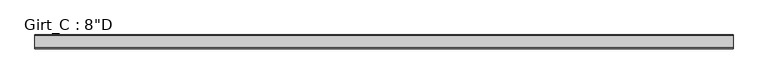
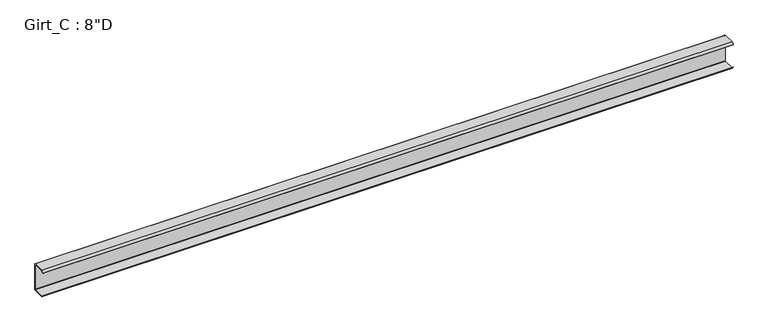
"""IFC4 building model written with IfcOpenShell, lengths in millimetres: beam geometry."""

import ifcopenshell
import ifcopenshell.guid

model = None  # the IFC model being written
_history = None  # IfcOwnerHistory: only IFC2X3 demands one
_inside = {}  # id of a spatial element -> (the spatial element, [elements in it])
_under = {}  # id of a project, library or spatial element -> (it, [spatial elements below it])
_declared = {}  # id of a project -> (the project, [libraries it declares])
_typed = {}  # id of a type object -> (the type object, [elements of that type])
_made_of = {}  # id of a material, layer set ... -> (it, [elements and type objects made of it])


def new_model(schema):
    """Start an empty IFC model of exactly this schema.

    Asked for "IFC4X3", IfcOpenShell would pick the latest addendum, in which some entities
    have other attributes; the version numbers below select the first issue.
    IFC2X3 requires an IfcOwnerHistory on every rooted entity: one is made here for all.
    """
    global model, _history
    if schema == "IFC4X3":
        model = ifcopenshell.file(schema_version=(4, 3, 0, 0))
    else:
        model = ifcopenshell.file(schema=schema)
    _inside.clear()
    _under.clear()
    _declared.clear()
    _typed.clear()
    _made_of.clear()
    _history = None
    if model.schema == "IFC2X3":
        org = make("IfcOrganization", Name="unknown")
        user = make(
            "IfcPersonAndOrganization",
            ThePerson=make("IfcPerson", FamilyName="unknown"),
            TheOrganization=org,
        )
        app = make(
            "IfcApplication",
            ApplicationDeveloper=org,
            Version="unknown",
            ApplicationFullName="unknown",
            ApplicationIdentifier="unknown",
        )
        _history = make(
            "IfcOwnerHistory",
            OwningUser=user,
            OwningApplication=app,
            ChangeAction="ADDED",
            CreationDate=0,
        )
    return model


def make(cls, **values):
    """One entity of the class cls with the attributes given. An attribute that is None is left unset."""
    return model.create_entity(
        cls, **{name: value for name, value in values.items() if value is not None}
    )


def rooted(cls, **values):
    """An entity with a GlobalId (a new one), such as an element, a storey or a relation."""
    return make(cls, GlobalId=ifcopenshell.guid.new(), OwnerHistory=_history, **values)


def si_unit(unit_type, name, prefix=None):
    """IfcSIUnit, for example si_unit("LENGTHUNIT", "METRE", prefix="MILLI")."""
    return make("IfcSIUnit", UnitType=unit_type, Prefix=prefix, Name=name)


def assignment(units):
    """IfcUnitAssignment: the units of a project."""
    return None if units is None else make("IfcUnitAssignment", Units=units)


def point(xyz):
    """IfcCartesianPoint."""
    return None if xyz is None else make("IfcCartesianPoint", Coordinates=xyz)


def direction(xyz):
    """IfcDirection."""
    return None if xyz is None else make("IfcDirection", DirectionRatios=xyz)


def frame(location, z_axis=None, x_axis=None):
    """IfcAxis2Placement3D, a coordinate frame: its origin and axes. An axis left out is left unset."""
    return make(
        "IfcAxis2Placement3D",
        Location=point(location),
        Axis=direction(z_axis),
        RefDirection=direction(x_axis),
    )


def frame_2d(location, x_axis=None):
    """IfcAxis2Placement2D, a coordinate frame in the plane: its origin and x axis."""
    return make(
        "IfcAxis2Placement2D", Location=point(location), RefDirection=direction(x_axis)
    )


def origin():
    """The frame at (0, 0, 0) with its axes left unset."""
    return frame((0.0, 0.0, 0.0))


def place(relative_to, where):
    """IfcLocalPlacement: puts the frame where relative to a parent placement (None: the world)."""
    return make(
        "IfcLocalPlacement", PlacementRelTo=relative_to, RelativePlacement=where
    )


def context(
    kind, dimensions, precision=None, world=None, true_north=None, identifier=None
):
    """IfcGeometricRepresentationContext, for example the 3D "Model" context."""
    return make(
        "IfcGeometricRepresentationContext",
        ContextIdentifier=identifier,
        ContextType=kind,
        CoordinateSpaceDimension=dimensions,
        Precision=precision,
        WorldCoordinateSystem=world,
        TrueNorth=true_north,
    )


def project(units=None, contexts=None):
    """IfcProject with its units and contexts."""
    return rooted(
        "IfcProject",
        Name="project",
        RepresentationContexts=contexts,
        UnitsInContext=assignment(units),
    )


def spatial(cls, under=None, at=None, **own):
    """A site, building, storey or space (cls), placed at a placement, below another one or the project."""
    s = rooted(cls, ObjectPlacement=at, **own)
    if under is not None:
        _under.setdefault(under.id(), (under, []))[1].append(s)
    return s


def polyline(points):
    """IfcPolyline through the points."""
    return make("IfcPolyline", Points=[point(p) for p in points])


def circle_curve(where, radius):
    """IfcCircle in the frame where."""
    return make("IfcCircle", Position=where, Radius=radius)


def trimmed(basis, trim1, trim2, sense, master):
    """IfcTrimmedCurve: the piece of a basis curve between two trims."""
    return make(
        "IfcTrimmedCurve",
        BasisCurve=basis,
        Trim1=trim1,
        Trim2=trim2,
        SenseAgreement=sense,
        MasterRepresentation=master,
    )


def segment(curve, same_sense, transition):
    """IfcCompositeCurveSegment."""
    return make(
        "IfcCompositeCurveSegment",
        Transition=transition,
        SameSense=same_sense,
        ParentCurve=curve,
    )


def composite_curve(segments, self_intersect=None):
    """IfcCompositeCurve: segments joined end to end."""
    return make("IfcCompositeCurve", Segments=segments, SelfIntersect=self_intersect)


def outline(outer, holes=None, kind="AREA"):
    """IfcArbitraryClosedProfileDef: a profile drawn as a closed curve; with holes, ...WithVoids."""
    if holes is None:
        return make("IfcArbitraryClosedProfileDef", ProfileType=kind, OuterCurve=outer)
    return make(
        "IfcArbitraryProfileDefWithVoids",
        ProfileType=kind,
        OuterCurve=outer,
        InnerCurves=holes,
    )


def extrude(swept, where, along, depth):
    """IfcExtrudedAreaSolid: the profile swept, set in the frame where, extruded along a direction by depth."""
    return make(
        "IfcExtrudedAreaSolid",
        SweptArea=swept,
        Position=where,
        ExtrudedDirection=direction(along),
        Depth=depth,
    )


def shape(context_of_items, identifier, shape_type, items):
    """IfcShapeRepresentation: the items that make up one representation, for example the "Body"."""
    return make(
        "IfcShapeRepresentation",
        ContextOfItems=context_of_items,
        RepresentationIdentifier=identifier,
        RepresentationType=shape_type,
        Items=items,
    )


def source(mapping_origin, context_of_items, identifier, shape_type, items):
    """IfcRepresentationMap: a shape defined once, which mapped items show again and again."""
    return make(
        "IfcRepresentationMap",
        MappingOrigin=mapping_origin,
        MappedRepresentation=shape(context_of_items, identifier, shape_type, items),
    )


def transform(
    local_origin,
    x_axis=None,
    y_axis=None,
    z_axis=None,
    scale=None,
    scale2=None,
    scale3=None,
    uniform=True,
):
    """IfcCartesianTransformationOperator3D, or its non-uniform kind. x_axis, y_axis, z_axis: its Axis1, 2, 3."""
    if uniform:
        return make(
            "IfcCartesianTransformationOperator3D",
            Axis1=direction(x_axis),
            Axis2=direction(y_axis),
            LocalOrigin=point(local_origin),
            Scale=scale,
            Axis3=direction(z_axis),
        )
    return make(
        "IfcCartesianTransformationOperator3DnonUniform",
        Axis1=direction(x_axis),
        Axis2=direction(y_axis),
        LocalOrigin=point(local_origin),
        Scale=scale,
        Axis3=direction(z_axis),
        Scale2=scale2,
        Scale3=scale3,
    )


def mapped(mapping_source, mapping_target):
    """IfcMappedItem: shows the shape of a source again, moved by a transform."""
    return make(
        "IfcMappedItem", MappingSource=mapping_source, MappingTarget=mapping_target
    )


def made_of(thing, what):
    """Note that an element or type object is made of a material, layer set ...; save() writes the relation."""
    if what is not None:
        _made_of.setdefault(what.id(), (what, []))[1].append(thing)
    return thing


def element(
    cls,
    number,
    at=None,
    inside=None,
    cuts=None,
    type_object=None,
    material=None,
    context=None,
    identifier="Body",
    shape_type=None,
    held_by="IfcProductDefinitionShape",
    body=None,
    shapes=None,
    **own,
):
    """One element of the class cls, such as IfcWall. Its Tag is "e" and its number.

    at: its placement. inside: the storey or other place that contains it. cuts: it is an
    opening in that element (IfcRelVoidsElement). A single representation is given by context,
    identifier, shape_type and body (its items); several are given by shapes. held_by: the class
    of the entity that holds the representations. save() writes the other relations.
    """
    e = rooted(cls, Tag="e%d" % number, ObjectPlacement=at, **own)
    if body is not None:
        shapes = [shape(context, identifier, shape_type, body)]
    if shapes is not None:
        e.Representation = make(held_by, Representations=shapes)
    if inside is not None:
        _inside.setdefault(inside.id(), (inside, []))[1].append(e)
    if cuts is not None:
        rooted(
            "IfcRelVoidsElement", RelatingBuildingElement=cuts, RelatedOpeningElement=e
        )
    if type_object is not None:
        _typed.setdefault(type_object.id(), (type_object, []))[1].append(e)
    return made_of(e, material)


def aggregate(whole, parts):
    """IfcRelAggregates: a whole, such as a stair, and the parts it consists of."""
    return rooted("IfcRelAggregates", RelatingObject=whole, RelatedObjects=parts)


def save(model, path):
    """Write the relations noted so far, then the file.

    IfcRelAggregates (storeys below a building ...), IfcRelContainedInSpatialStructure (elements
    in a storey), IfcRelDefinesByType, IfcRelAssociatesMaterial and IfcRelDeclares: one each for
    every whole, place, type object, material and project.
    """
    for whole, parts in _under.values():
        aggregate(whole, parts)
    for where, things in _inside.values():
        rooted(
            "IfcRelContainedInSpatialStructure",
            RelatedElements=things,
            RelatingStructure=where,
        )
    for kind, things in _typed.values():
        rooted("IfcRelDefinesByType", RelatedObjects=things, RelatingType=kind)
    for what, things in _made_of.values():
        rooted("IfcRelAssociatesMaterial", RelatedObjects=things, RelatingMaterial=what)
    for by, libraries in _declared.values():
        rooted("IfcRelDeclares", RelatingContext=by, RelatedDefinitions=libraries)
    model.write(path)


def beam_0a0f1977(model_context):
    return source(origin(), model_context, "Body", "SweptSolid", [
        extrude(outline(composite_curve([segment(polyline([(-87.5109375, 101.6), (-3.3734375, 101.6)]), True, "CONTINUOUS"), segment(trimmed(circle_curve(frame_2d((-3.3734375, 96.8375)), 4.7625), [point((-3.3734375, 101.6))], [point((1.3890625, 96.8375))], False, "CARTESIAN"), True, "CONTINUOUS"), segment(polyline([(1.3890625, 96.8375), (1.3890625, -96.8375)]), True, "CONTINUOUS"), segment(trimmed(circle_curve(frame_2d((-3.3734375, -96.8375)), 4.7625), [point((1.3890625, -96.8375))], [point((-3.3734375, -101.6))], False, "CARTESIAN"), True, "CONTINUOUS"), segment(polyline([(-3.3734375, -101.6), (-87.5109375, -101.6), (-99.7792647, -86.979177), (-97.6510975, -85.1934327), (-86.2154765, -98.821875), (-3.2694106, -98.821875)]), True, "CONTINUOUS"), segment(trimmed(circle_curve(frame_2d((-3.3748024, -96.8389339)), 1.9857399), [point((-3.2694106, -98.821875))], [point((-1.3890625, -96.8389339))], True, "CARTESIAN"), True, "CONTINUOUS"), segment(polyline([(-1.3890625, -96.8389339), (-1.3890625, 96.8381931)]), True, "CONTINUOUS"), segment(trimmed(circle_curve(frame_2d((-3.3741066, 96.8381931)), 1.9850441), [point((-1.3890625, 96.8381931))], [point((-3.3005807, 98.821875))], True, "CARTESIAN"), True, "CONTINUOUS"), segment(polyline([(-3.3005807, 98.821875), (-86.2154765, 98.821875), (-97.6278742, 85.221109), (-99.7560415, 87.0068534), (-87.5109375, 101.6)]), True, "CONTINUOUS")], self_intersect=False)), frame((-2543.96875, 0.0, 0.0), z_axis=(1.0, 0.0, 0.0), x_axis=(0.0, 1.0, 0.0)), (0.0, 0.0, 1.0), 5015.8015),
    ])


if __name__ == "__main__":
    model = new_model("IFC4")
    model_context = context("Model", 3, world=origin())
    ifc_project = project(units=[si_unit("LENGTHUNIT", "METRE", prefix="MILLI")], contexts=[model_context])
    site = spatial("IfcSite", under=ifc_project)
    building = spatial("IfcBuilding", under=site)
    placement = place(None, origin())
    beam_shape = beam_0a0f1977(model_context)
    element("IfcBeam", 1, ObjectType="Girt_C : 8\"D", at=placement, inside=building, context=model_context, shape_type="MappedRepresentation", body=[
        mapped(beam_shape, transform((0.0, 0.0, 0.0), x_axis=(1.0, 0.0, 0.0), y_axis=(0.0, 1.0, 0.0), z_axis=(0.0, 0.0, 1.0))),
    ])
    save(model, "model.ifc")

# Revit data of these elements
# Type "Girt_C : 8\"D"
#   half leg = 0' - 1 3/4"
#   Web_Thickness = 0' - 0 7/64"
#   Length [instance default] = 10' - 0"
#   Leg_1 = 0' - 3 1/2"
#   Height = 0' - 8"
#   Structural Material [instance default] = none
# Element 1 (IfcBeam, "Girt_C : 8\"D")
#   Structural Material = CEE' SECTION (8.0x3.5C - SEE STRUCT. DWGS)
#   Materials on its faces: "CEE' SECTION (8.0x3.5C - SEE STRUCT. DWGS)"
# Materials
#   "CEE' SECTION (8.0x3.5C - SEE STRUCT. DWGS)": class "Metal", colour RGB 137 146 153, transparency 0, Description = "Steel, mill finish", Cost = 0
